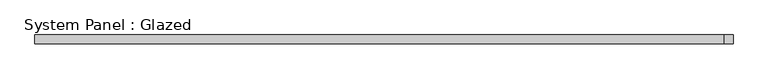
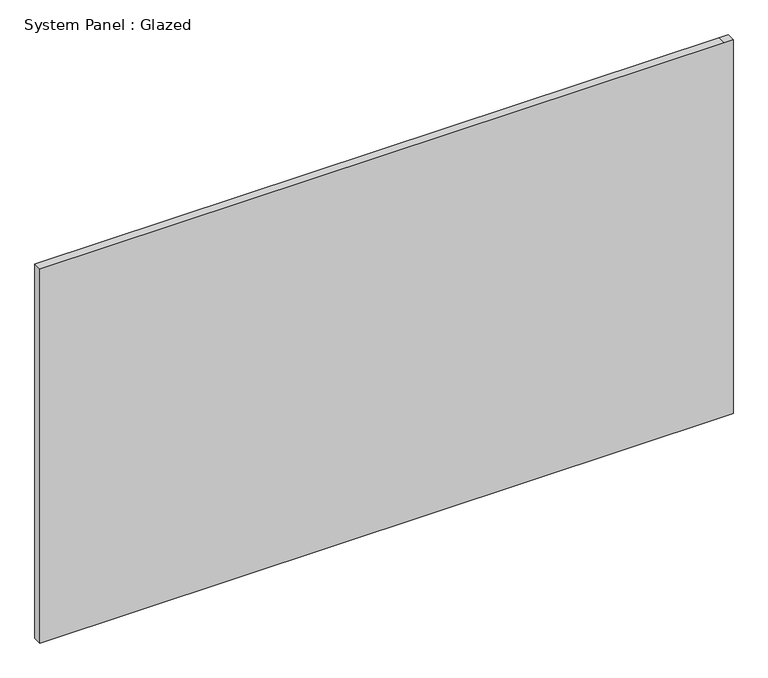
"""IFC4 building model written with IfcOpenShell, lengths in millimetres: plate geometry, System Panel : Glazed."""

from ifc_helpers import new_model, si_unit, frame, origin, place, context, project, spatial, polyline, outline, extrude, source, transform, mapped, element, save


def system_panel_glazed_75599714(model_context):
    return source(origin(), model_context, "Body", "SweptSolid", [
        extrude(outline(polyline([(0.0, -1012.825), (0.0, 987.425), (0.0, 1012.825), (1155.7, 1012.825), (1155.7, 987.425), (1155.7, -1012.825), (0.0, -1012.825)])), frame((0.0, -44.45, 0.0), z_axis=(0.0, 1.0, 0.0), x_axis=(0.0, 0.0, 1.0)), (0.0, 0.0, 1.0), 25.4),
    ])


if __name__ == "__main__":
    model = new_model("IFC4")
    model_context = context("Model", 3, world=origin())
    ifc_project = project(units=[si_unit("LENGTHUNIT", "METRE", prefix="MILLI")], contexts=[model_context])
    site = spatial("IfcSite", under=ifc_project)
    building = spatial("IfcBuilding", under=site)
    placement = place(None, origin())
    system_panel_glazed_shape = system_panel_glazed_75599714(model_context)
    element("IfcPlate", 1, ObjectType="System Panel : Glazed", at=placement, inside=building, context=model_context, shape_type="MappedRepresentation", body=[
        mapped(system_panel_glazed_shape, transform((0.0, 0.0, 0.0), x_axis=(1.0, 0.0, 0.0), y_axis=(0.0, 1.0, 0.0), z_axis=(0.0, 0.0, 1.0))),
    ])
    save(model, "model.ifc")

# Revit data of these elements
# Element 1 (IfcPlate, "System Panel : Glazed")
#   Materials on its faces: "Glass"
# Materials
#   "Glass": class "Glass", colour RGB 0 128 192, transparency 0.75
